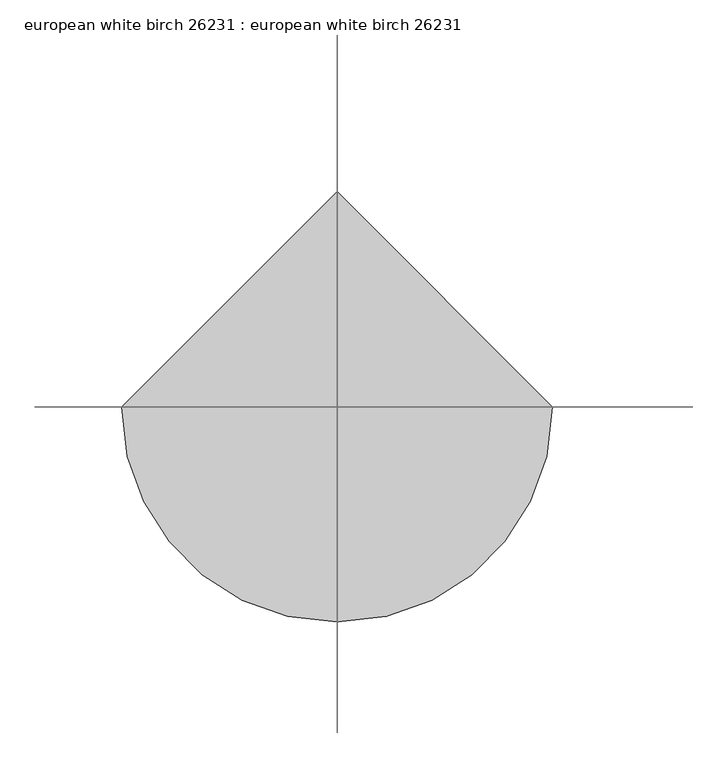
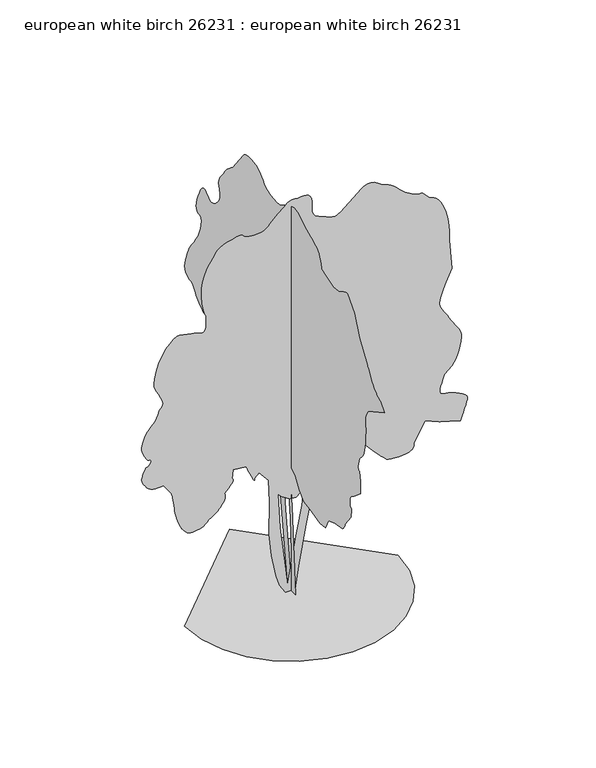
"""IFC4 building model written with IfcOpenShell, lengths in millimetres: proxy geometry, european white birch 26231 : european white birch 26231."""

import ifcopenshell
import ifcopenshell.guid

model = None  # the IFC model being written
_history = None  # IfcOwnerHistory: only IFC2X3 demands one
_inside = {}  # id of a spatial element -> (the spatial element, [elements in it])
_under = {}  # id of a project, library or spatial element -> (it, [spatial elements below it])
_declared = {}  # id of a project -> (the project, [libraries it declares])
_typed = {}  # id of a type object -> (the type object, [elements of that type])
_made_of = {}  # id of a material, layer set ... -> (it, [elements and type objects made of it])


def new_model(schema):
    """Start an empty IFC model of exactly this schema.

    Asked for "IFC4X3", IfcOpenShell would pick the latest addendum, in which some entities
    have other attributes; the version numbers below select the first issue.
    IFC2X3 requires an IfcOwnerHistory on every rooted entity: one is made here for all.
    """
    global model, _history
    if schema == "IFC4X3":
        model = ifcopenshell.file(schema_version=(4, 3, 0, 0))
    else:
        model = ifcopenshell.file(schema=schema)
    _inside.clear()
    _under.clear()
    _declared.clear()
    _typed.clear()
    _made_of.clear()
    _history = None
    if model.schema == "IFC2X3":
        org = make("IfcOrganization", Name="unknown")
        user = make(
            "IfcPersonAndOrganization",
            ThePerson=make("IfcPerson", FamilyName="unknown"),
            TheOrganization=org,
        )
        app = make(
            "IfcApplication",
            ApplicationDeveloper=org,
            Version="unknown",
            ApplicationFullName="unknown",
            ApplicationIdentifier="unknown",
        )
        _history = make(
            "IfcOwnerHistory",
            OwningUser=user,
            OwningApplication=app,
            ChangeAction="ADDED",
            CreationDate=0,
        )
    return model


def make(cls, **values):
    """One entity of the class cls with the attributes given. An attribute that is None is left unset."""
    return model.create_entity(
        cls, **{name: value for name, value in values.items() if value is not None}
    )


def rooted(cls, **values):
    """An entity with a GlobalId (a new one), such as an element, a storey or a relation."""
    return make(cls, GlobalId=ifcopenshell.guid.new(), OwnerHistory=_history, **values)


def si_unit(unit_type, name, prefix=None):
    """IfcSIUnit, for example si_unit("LENGTHUNIT", "METRE", prefix="MILLI")."""
    return make("IfcSIUnit", UnitType=unit_type, Prefix=prefix, Name=name)


def assignment(units):
    """IfcUnitAssignment: the units of a project."""
    return None if units is None else make("IfcUnitAssignment", Units=units)


def point(xyz):
    """IfcCartesianPoint."""
    return None if xyz is None else make("IfcCartesianPoint", Coordinates=xyz)


def direction(xyz):
    """IfcDirection."""
    return None if xyz is None else make("IfcDirection", DirectionRatios=xyz)


def frame(location, z_axis=None, x_axis=None):
    """IfcAxis2Placement3D, a coordinate frame: its origin and axes. An axis left out is left unset."""
    return make(
        "IfcAxis2Placement3D",
        Location=point(location),
        Axis=direction(z_axis),
        RefDirection=direction(x_axis),
    )


def origin():
    """The frame at (0, 0, 0) with its axes left unset."""
    return frame((0.0, 0.0, 0.0))


def place(relative_to, where):
    """IfcLocalPlacement: puts the frame where relative to a parent placement (None: the world)."""
    return make(
        "IfcLocalPlacement", PlacementRelTo=relative_to, RelativePlacement=where
    )


def context(
    kind, dimensions, precision=None, world=None, true_north=None, identifier=None
):
    """IfcGeometricRepresentationContext, for example the 3D "Model" context."""
    return make(
        "IfcGeometricRepresentationContext",
        ContextIdentifier=identifier,
        ContextType=kind,
        CoordinateSpaceDimension=dimensions,
        Precision=precision,
        WorldCoordinateSystem=world,
        TrueNorth=true_north,
    )


def project(units=None, contexts=None):
    """IfcProject with its units and contexts."""
    return rooted(
        "IfcProject",
        Name="project",
        RepresentationContexts=contexts,
        UnitsInContext=assignment(units),
    )


def spatial(cls, under=None, at=None, **own):
    """A site, building, storey or space (cls), placed at a placement, below another one or the project."""
    s = rooted(cls, ObjectPlacement=at, **own)
    if under is not None:
        _under.setdefault(under.id(), (under, []))[1].append(s)
    return s


def point_list(points):
    """IfcCartesianPointList2D or 3D."""
    cls = (
        "IfcCartesianPointList2D" if len(points[0]) == 2 else "IfcCartesianPointList3D"
    )
    return make(cls, CoordList=points)


def triangles(points, corners, closed=None, point_numbers=None):
    """IfcTriangulatedFaceSet: each triangle names its three corners, points numbered from 1."""
    return make(
        "IfcTriangulatedFaceSet",
        Coordinates=point_list(points),
        Closed=closed,
        CoordIndex=corners,
        PnIndex=point_numbers,
    )


def shape(context_of_items, identifier, shape_type, items):
    """IfcShapeRepresentation: the items that make up one representation, for example the "Body"."""
    return make(
        "IfcShapeRepresentation",
        ContextOfItems=context_of_items,
        RepresentationIdentifier=identifier,
        RepresentationType=shape_type,
        Items=items,
    )


def source(mapping_origin, context_of_items, identifier, shape_type, items):
    """IfcRepresentationMap: a shape defined once, which mapped items show again and again."""
    return make(
        "IfcRepresentationMap",
        MappingOrigin=mapping_origin,
        MappedRepresentation=shape(context_of_items, identifier, shape_type, items),
    )


def transform(
    local_origin,
    x_axis=None,
    y_axis=None,
    z_axis=None,
    scale=None,
    scale2=None,
    scale3=None,
    uniform=True,
):
    """IfcCartesianTransformationOperator3D, or its non-uniform kind. x_axis, y_axis, z_axis: its Axis1, 2, 3."""
    if uniform:
        return make(
            "IfcCartesianTransformationOperator3D",
            Axis1=direction(x_axis),
            Axis2=direction(y_axis),
            LocalOrigin=point(local_origin),
            Scale=scale,
            Axis3=direction(z_axis),
        )
    return make(
        "IfcCartesianTransformationOperator3DnonUniform",
        Axis1=direction(x_axis),
        Axis2=direction(y_axis),
        LocalOrigin=point(local_origin),
        Scale=scale,
        Axis3=direction(z_axis),
        Scale2=scale2,
        Scale3=scale3,
    )


def mapped(mapping_source, mapping_target):
    """IfcMappedItem: shows the shape of a source again, moved by a transform."""
    return make(
        "IfcMappedItem", MappingSource=mapping_source, MappingTarget=mapping_target
    )


def made_of(thing, what):
    """Note that an element or type object is made of a material, layer set ...; save() writes the relation."""
    if what is not None:
        _made_of.setdefault(what.id(), (what, []))[1].append(thing)
    return thing


def element(
    cls,
    number,
    at=None,
    inside=None,
    cuts=None,
    type_object=None,
    material=None,
    context=None,
    identifier="Body",
    shape_type=None,
    held_by="IfcProductDefinitionShape",
    body=None,
    shapes=None,
    **own,
):
    """One element of the class cls, such as IfcWall. Its Tag is "e" and its number.

    at: its placement. inside: the storey or other place that contains it. cuts: it is an
    opening in that element (IfcRelVoidsElement). A single representation is given by context,
    identifier, shape_type and body (its items); several are given by shapes. held_by: the class
    of the entity that holds the representations. save() writes the other relations.
    """
    e = rooted(cls, Tag="e%d" % number, ObjectPlacement=at, **own)
    if body is not None:
        shapes = [shape(context, identifier, shape_type, body)]
    if shapes is not None:
        e.Representation = make(held_by, Representations=shapes)
    if inside is not None:
        _inside.setdefault(inside.id(), (inside, []))[1].append(e)
    if cuts is not None:
        rooted(
            "IfcRelVoidsElement", RelatingBuildingElement=cuts, RelatedOpeningElement=e
        )
    if type_object is not None:
        _typed.setdefault(type_object.id(), (type_object, []))[1].append(e)
    return made_of(e, material)


def aggregate(whole, parts):
    """IfcRelAggregates: a whole, such as a stair, and the parts it consists of."""
    return rooted("IfcRelAggregates", RelatingObject=whole, RelatedObjects=parts)


def save(model, path):
    """Write the relations noted so far, then the file.

    IfcRelAggregates (storeys below a building ...), IfcRelContainedInSpatialStructure (elements
    in a storey), IfcRelDefinesByType, IfcRelAssociatesMaterial and IfcRelDeclares: one each for
    every whole, place, type object, material and project.
    """
    for whole, parts in _under.values():
        aggregate(whole, parts)
    for where, things in _inside.values():
        rooted(
            "IfcRelContainedInSpatialStructure",
            RelatedElements=things,
            RelatingStructure=where,
        )
    for kind, things in _typed.values():
        rooted("IfcRelDefinesByType", RelatedObjects=things, RelatingType=kind)
    for what, things in _made_of.values():
        rooted("IfcRelAssociatesMaterial", RelatedObjects=things, RelatingMaterial=what)
    for by, libraries in _declared.values():
        rooted("IfcRelDeclares", RelatingContext=by, RelatedDefinitions=libraries)
    model.write(path)


def european_white_birch_26231_european_white_birch_26231_e71fde4f(model_context):
    return source(origin(), model_context, "Body", "Tessellation", [
        triangles([(27.394651, 0.0040504, 0.0028461), (-40.6021365, 0.0040504, 0.0028461), (-85.9329906, 0.0040461, 71.7768143), (-112.3759078, 0.0040411, 154.8832968), (-146.3742959, 0.004031, 324.873484), (-165.2619874, 0.0040206, 498.6424559), (-161.4844927, 0.004006, 744.1841543), (-169.039464, 0.0039956, 917.9531261), (-237.036004, 0.0039907, 1001.059318), (-271.0331294, 0.0039925, 970.840959), (-270.3066839, 0.0039929, 963.7695883), (-270.075557, 0.0039933, 957.9860023), (-270.8350129, 0.0039934, 954.7830729), (-273.0829134, 0.0039934, 955.4434977), (-277.3120158, 0.0039931, 961.2575323), (-284.0176021, 0.0039923, 973.5155777), (-293.700078, 0.0039911, 993.5053459), (-303.821971, 0.0039898, 1015.3671656), (-311.7620024, 0.0039888, 1032.8676962), (-317.8859382, 0.003988, 1046.7335649), (-322.5544759, 0.0039873, 1057.6911083), (-326.1333272, 0.0039868, 1066.4693516), (-328.985733, 0.0039864, 1073.7921604), (-331.4749343, 0.0039859, 1080.3885601), (-429.6916137, 0.0039853, 1091.7220253), (-437.2481292, 0.0039893, 1023.7262484), (-433.293356, 0.0039894, 1022.0295496), (-429.9024656, 0.0039896, 1019.8705244), (-427.631674, 0.0039898, 1016.7869917), (-427.0500235, 0.00399, 1012.316625), (-428.7111866, 0.0039904, 1005.9945545), (-433.1841331, 0.0039909, 997.3610699), (-441.0251152, 0.0039916, 985.9513739), (-450.1868743, 0.0039923, 973.9905487), (-458.3606123, 0.0039929, 963.8127542), (-465.7062758, 0.0039934, 955.1234591), (-472.3915509, 0.0039939, 947.6228268), (-478.5815437, 0.0039942, 941.0162533), (-484.4387807, 0.0039946, 935.0015768), (-490.1334549, 0.003995, 929.2865913), (-488.5815147, 0.0039955, 919.5735941), (-487.4232642, 0.0039961, 909.8581261), (-487.0600596, 0.0039967, 900.1451288), (-487.8880978, 0.0039973, 890.4322042), (-490.2985611, 0.0039979, 880.7167362), (-494.6927333, 0.0039984, 871.003739), (-501.4669201, 0.003999, 861.2908144), (-508.8125836, 0.0039996, 851.763271), (-515.365781, 0.0040001, 842.4363693), (-522.1831338, 0.0040007, 833.0409399), (-530.3212998, 0.0040013, 823.3152981), (-540.8394442, 0.0040019, 812.9977592), (-554.7941883, 0.0040026, 801.8192265), (-573.2396831, 0.0040033, 789.5154716), (-592.1829672, 0.0040041, 776.4217941), (-607.7557085, 0.0040048, 763.3916302), (-621.2152067, 0.0040056, 750.9583048), (-633.8135656, 0.0040063, 739.6477306), (-646.8107374, 0.0040068, 729.9880732), (-661.4563551, 0.0040073, 722.5103319), (-679.0128416, 0.0040076, 717.742745), (-697.3389759, 0.0040078, 714.6033291), (-713.6812923, 0.0040079, 712.0582083), (-728.3751629, 0.004008, 710.7044392), (-741.7431696, 0.004008, 711.1337008), (-754.1231552, 0.0040078, 713.9429043), (-765.842716, 0.0040075, 719.7239468), (-777.229521, 0.0040069, 729.0736668), (-788.1109062, 0.0040062, 740.6941784), (-798.1336956, 0.0040055, 753.1071562), (-807.361548, 0.0040047, 766.6428125), (-815.8629187, 0.0040037, 781.6313599), (-823.7064079, 0.0040028, 798.4029379), (-830.9530586, 0.0040016, 817.2929186), (-837.6713259, 0.0040004, 838.6238113), (-843.4955343, 0.0039992, 858.8117506), (-848.1996077, 0.0039982, 875.2328413), (-852.042687, 0.0039973, 889.6727303), (-855.291326, 0.0039965, 903.9119774), (-858.2097525, 0.0039955, 919.7387003), (-861.0621946, 0.0039944, 938.9334589), (-864.1127352, 0.0039929, 963.2844435), (-867.2419773, 0.0039915, 988.1637388), (-870.1706503, 0.0039902, 1008.2856211), (-872.9341444, 0.0039893, 1024.4425564), (-875.5681406, 0.0039885, 1037.4270109), (-878.1005442, 0.0039879, 1048.0315235), (-880.566818, 0.0039873, 1057.0510311), (-883.0001724, 0.0039869, 1065.2781452), (-939.6650276, 0.0039821, 1144.6073874), (-960.6453604, 0.0039822, 1143.9037966), (-981.2295691, 0.0039822, 1143.8250223), (-1001.0212389, 0.0039821, 1145.0035841), (-1019.6216297, 0.0039819, 1148.0668419), (-1036.6370882, 0.0039816, 1153.6396122), (-1051.6713449, 0.0039811, 1162.3517984), (-1064.3255871, 0.0039803, 1174.8282898), (-1074.7447186, 0.0039795, 1188.5290524), (-1083.3781305, 0.0039788, 1200.7108669), (-1090.2945688, 0.0039781, 1211.7014025), (-1095.5600178, 0.0039775, 1221.8335602), (-1099.2379183, 0.003977, 1231.4371891), (-1101.3968708, 0.0039764, 1240.842865), (-1102.1004616, 0.0039758, 1250.3805096), (-1100.4266539, 0.0039751, 1261.9120731), (-1096.1086035, 0.0039743, 1276.0193516), (-1090.2056934, 0.0039734, 1291.1195927), (-1083.7743999, 0.0039725, 1305.6229225), (-1077.8714172, 0.0039718, 1317.9470249), (-1073.5534395, 0.0039713, 1326.5043514), (-1071.8795591, 0.0039711, 1329.7098244), (-1068.9941248, 0.003971, 1330.8324303), (-1061.7475468, 0.0039708, 1334.0708954), (-1052.2555389, 0.0039705, 1339.2246506), (-1042.6289463, 0.0039701, 1346.0979229), (-1034.9860989, 0.0039696, 1354.4899979), (-1031.4402397, 0.003969, 1364.2029224), (-1034.1046846, 0.0039684, 1375.0412144), (-1039.5885796, 0.003968, 1382.3080673), (-1043.7516249, 0.0039679, 1383.6975174), (-1047.5844578, 0.0039679, 1382.5722954), (-1052.0777155, 0.003968, 1382.3080673), (-1058.224506, 0.0039677, 1386.2730869), (-1067.012923, 0.003967, 1397.8376427), (-1079.4360746, 0.0039657, 1420.3699883), (-1091.9252106, 0.0039642, 1445.7800652), (-1100.2513739, 0.003963, 1465.4371502), (-1104.4144192, 0.003962, 1481.9243706), (-1104.4144192, 0.0039611, 1497.8171505), (-1100.2513739, 0.00396, 1515.6910595), (-1091.9252106, 0.0039587, 1538.1268993), (-1079.4360746, 0.0039569, 1567.6974781), (-1064.2798777, 0.0039552, 1597.0701038), (-1048.399815, 0.0039538, 1619.0410011), (-1032.4536953, 0.0039528, 1636.3867447), (-1017.0993999, 0.0039519, 1651.8833279), (-1003.0024406, 0.0039509, 1668.3044186), (-990.8230968, 0.0039497, 1688.4261555), (-981.2193953, 0.0039481, 1715.0224972), (-972.0448826, 0.0039467, 1739.5715801), (-961.9458624, 0.0039458, 1754.6033661), (-952.7714224, 0.0039452, 1764.484013), (-946.3731211, 0.0039446, 1773.5695049), (-944.597648, 0.0039439, 1786.2238197), (-949.3017941, 0.0039427, 1806.8080284), (-962.3294146, 0.0039407, 1839.683202), (-979.0807177, 0.0039386, 1873.8004509), (-993.1903942, 0.0039372, 1898.4714741), (-1003.8609638, 0.003936, 1918.5805664), (-1010.3049019, 0.0039348, 1939.0224873), (-1011.7248007, 0.0039332, 1964.6841476), (-1007.3305922, 0.0039311, 2000.4549294), (-996.3298101, 0.0039281, 2051.2269756), (-977.7827591, 0.0039247, 2108.3871494), (-952.959347, 0.0039217, 2159.268346), (-924.3666155, 0.0039191, 2202.6819752), (-894.5216349, 0.003917, 2237.4394466), (-865.9313742, 0.0039155, 2262.3517342), (-841.1054186, 0.0039147, 2276.2302475), (-822.560911, 0.0039146, 2277.8813095), (-705.4567944, 0.0039161, 2251.4372841), (-691.5452162, 0.0039165, 2245.6562416), (-676.5135029, 0.0039168, 2239.8751991), (-661.5453032, 0.003917, 2236.8678246), (-647.8343668, 0.0039169, 2239.4104019), (-636.5669586, 0.0039162, 2250.281686), (-628.9342123, 0.0039149, 2272.2525833), (-626.1275522, 0.0039128, 2308.1021393), (-626.6101536, 0.0039108, 2340.8655464), (-628.1519199, 0.0039099, 2356.9793884), (-630.8849653, 0.0039094, 2364.3021973), (-634.9362442, 0.003909, 2370.7004986), (-640.4429575, 0.0039082, 2384.0379112), (-647.5371466, 0.0039066, 2412.1786354), (-656.3459112, 0.0039035, 2462.9810577), (-661.9085077, 0.0038998, 2524.9316368), (-660.1355782, 0.0038965, 2581.121521), (-652.4800135, 0.0038935, 2631.3882202), (-640.3997915, 0.0038909, 2675.5079109), (-625.3451872, 0.0038886, 2713.2524094), (-608.7691641, 0.0038868, 2744.4943977), (-592.1271203, 0.0038853, 2768.9545326), (-577.5017776, 0.0038841, 2789.7061729), (-564.8602163, 0.0038829, 2809.5183357), (-552.480267, 0.0038818, 2827.9332001), (-538.6474268, 0.0038808, 2844.519397), (-521.6421421, 0.00388, 2858.7688179), (-499.7473303, 0.0038793, 2870.2750923), (-471.2460176, 0.0038788, 2878.5045319), (-442.3357547, 0.0038784, 2885.0579109), (-419.4402045, 0.003878, 2891.1537598), (-401.1674463, 0.0038777, 2895.8528915), (-386.135733, 0.0038776, 2898.2405365), (-372.9506003, 0.0038776, 2897.4022156), (-360.2302649, 0.0038779, 2892.3984512), (-346.5853855, 0.0038786, 2882.2891846), (-328.0611892, 0.0038792, 2871.5959419), (-303.3901842, 0.0038796, 2865.1951698), (-275.2190476, 0.0038797, 2862.7566559), (-246.1878799, 0.0038796, 2863.9757675), (-218.9407967, 0.0038794, 2868.471714), (-196.1211867, 0.0038789, 2875.9392815), (-180.3721843, 0.0038783, 2886.0738373), (-168.3897398, 0.0038776, 2898.2405365), (-155.2838538, 0.0038768, 2911.7277946), (-141.3189358, 0.0038759, 2926.0280846), (-126.7594139, 0.0038751, 2940.5568489), (-111.8694252, 0.0038742, 2954.8571388), (-96.9134068, 0.0038734, 2968.344397), (-82.1555049, 0.0038727, 2980.5110962), (-68.1573178, 0.003872, 2992.5760574), (-54.8202912, 0.0038712, 3005.3776016), (-41.4169714, 0.0038705, 3017.7727753), (-27.2206609, 0.0038698, 3028.6694939), (-11.5045701, 0.0038693, 3036.8989334), (6.4582013, 0.0038691, 3041.3693001), (27.394651, 0.0038691, 3040.9629295), (49.9498399, 0.0038692, 3039.6420799), (71.8443792, 0.0038691, 3040.7344551), (92.4173513, 0.003869, 3041.9535667), (111.007859, 0.0038691, 3041.0390877), (126.954987, 0.0038694, 3035.7812691), (139.5983468, 0.0038701, 3023.8942039), (148.2767597, 0.0038713, 3003.1678528), (152.1975051, 0.0038729, 2976.7517326), (152.8144732, 0.0038745, 2949.9039528), (152.8363106, 0.0038761, 2923.6913086), (154.9729534, 0.0038776, 2899.0276978), (161.9335751, 0.0038789, 2876.9552078), (176.4270581, 0.00388, 2858.4641853), (201.1628484, 0.0038808, 2844.519397), (230.392387, 0.0038815, 2832.759359), (256.9132791, 0.0038822, 2821.2022156), (281.2515464, 0.0038828, 2811.4231613), (303.9388244, 0.0038832, 2804.9971001), (325.5034238, 0.0038833, 2803.5492233), (346.4736554, 0.0038829, 2808.6291458), (367.3752866, 0.0038822, 2821.8626404), (518.4798351, 0.0038745, 2950.2850342), (522.0028032, 0.0038744, 2952.6726791), (531.8706965, 0.003874, 2958.2098412), (547.0243501, 0.0038737, 2964.5597443), (566.409613, 0.0038734, 2969.309745), (588.9648133, 0.0038733, 2970.1224861), (613.6332567, 0.0038737, 2964.5597443), (639.3609015, 0.0038745, 2950.2850342), (662.9625858, 0.0038755, 2934.3845512), (682.9295357, 0.0038761, 2923.8183357), (700.7171127, 0.0038765, 2916.096714), (717.7757372, 0.003877, 2908.7053047), (735.5633869, 0.0038775, 2899.1294357), (755.5303368, 0.0038784, 2884.8800148), (779.1320211, 0.0038797, 2863.4170807), (802.6904669, 0.003881, 2840.7347443), (822.3475519, 0.0038821, 2823.6151497), (839.2969534, 0.0038828, 2810.6612892), (854.7274069, 0.0038834, 2800.5011536), (869.8277206, 0.0038839, 2791.7130272), (885.7865576, 0.0038845, 2782.9246101), (903.7925806, 0.0038851, 2772.7391853), (921.1153605, 0.0038856, 2764.6873512), (935.0701773, 0.0038857, 2761.4360962), (946.9090622, 0.0038858, 2760.445459), (957.8894966, 0.0038859, 2759.1246094), (969.2661278, 0.0038861, 2754.908297), (982.2963644, 0.0038867, 2745.1801117), (998.2323103, 0.0038878, 2727.4000923), (1015.8421366, 0.0038888, 2709.5947838), (1033.1877348, 0.0038895, 2698.6471962), (1050.4673487, 0.00389, 2690.3415985), (1067.8790766, 0.0038906, 2680.4608063), (1085.6209442, 0.0038915, 2664.7382195), (1103.8937387, 0.0038931, 2639.0081039), (1122.890399, 0.0038954, 2598.9776985), (1139.5654713, 0.0038982, 2552.2671776), (1151.2850321, 0.0039008, 2508.9526703), (1158.8719963, 0.0039032, 2468.4345039), (1163.1569818, 0.0039055, 2430.1618401), (1164.9629036, 0.0039077, 2393.5757011), (1165.1152925, 0.0039098, 2358.1121681), (1164.4447666, 0.0039119, 2323.2125542), (1183.3322039, 0.0039254, 2096.5583656), (1160.8760891, 0.0039282, 2049.0019661), (1139.6746943, 0.003931, 2002.6697651), (1120.9853554, 0.0039336, 1958.7811649), (1106.0628651, 0.003936, 1918.5603642), (1096.1619432, 0.0039381, 1883.2289452), (1092.5373825, 0.0039398, 1854.0112518), (1096.4489897, 0.0039411, 1832.1266865), (1105.2043419, 0.0039422, 1814.483868), (1115.1484297, 0.0039432, 1796.9070339), (1126.0856981, 0.0039443, 1778.9975166), (1137.8154327, 0.0039454, 1760.364061), (1150.1394625, 0.0039466, 1740.6053833), (1162.8597616, 0.0039479, 1719.327903), (1175.7782318, 0.0039492, 1696.1351326), (1190.083536, 0.0039507, 1672.4673912), (1206.0423002, 0.003952, 1649.7243027), (1222.0671215, 0.0039534, 1627.4433952), (1236.5705967, 0.0039547, 1605.1651039), (1247.9700462, 0.003956, 1582.42187), (1254.6782124, 0.0039574, 1558.7541286), (1255.1075466, 0.0039589, 1533.6996986), (1250.5482319, 0.0039606, 1505.3836945), (1243.6089752, 0.0039625, 1473.6972565), (1234.6884441, 0.0039645, 1440.8220829), (1224.1805099, 0.0039664, 1408.9400173), (1212.4837675, 0.0039681, 1380.2278164), (1199.9971024, 0.0039695, 1356.867469), (1187.1091536, 0.0039704, 1341.0432896), (1175.1508718, 0.003971, 1330.4793995), (1164.9730774, 0.0039716, 1321.3074303), (1156.2837095, 0.0039721, 1313.2887337), (1148.7831499, 0.0039725, 1306.1970154), (1142.1765764, 0.0039729, 1299.7962433), (1136.1618999, 0.0039732, 1293.8602684), (1130.4468418, 0.0039736, 1288.1553841), (1119.2784828, 0.0039753, 1259.9842838), (1109.1032318, 0.0039769, 1232.7706833), (1100.9092552, 0.0039784, 1207.4723728), (1095.6869722, 0.0039797, 1185.0492502), (1094.4322523, 0.0039808, 1166.4589605), (1098.1329712, 0.0039817, 1152.6591488), (1107.7799114, 0.0039821, 1144.6073874), (1119.8855679, 0.0039824, 1140.5992744), (1130.6017742, 0.0039825, 1137.9779955), (1140.3909296, 0.0039826, 1136.2812241), (1149.7203747, 0.0039827, 1135.0493225), (1159.0472763, 0.0039828, 1133.8148775), (1168.8389751, 0.0039829, 1132.1181787), (1179.5551815, 0.003983, 1129.4968998), (1194.774892, 0.0039834, 1124.1121267), (1215.7451237, 0.0039839, 1115.0925465), (1239.4230389, 0.0039846, 1103.4288689), (1262.7705963, 0.0039854, 1090.1142019), (1282.7503361, 0.0039862, 1076.1391829), (1296.3189846, 0.003987, 1062.4917601), (1300.4363205, 0.0039877, 1050.1676577), (1297.6066967, 0.0039886, 1036.4135553), (1292.5953747, 0.0039897, 1018.2957659), (1285.7677391, 0.0039909, 996.5457127), (1277.4848145, 0.0039924, 971.8848633), (1268.1122761, 0.003994, 945.0472572), (1258.0131832, 0.0039957, 916.7542168), (1247.5510311, 0.0039974, 887.732151), (1088.8924742, 0.0039947, 933.063541), (986.8988451, 0.003992, 978.394931), (903.7925806, 0.0040008, 831.069912), (903.6808142, 0.0040014, 821.3899796), (902.9112391, 0.0040019, 811.9056021), (900.8182709, 0.0040025, 802.8200375), (896.744101, 0.004003, 794.328768), (890.0258337, 0.0040035, 786.6300373), (880.0029716, 0.0040039, 779.9244873), (866.0151627, 0.0040042, 774.4050568), (846.3124409, 0.0040044, 770.254656), (821.2578655, 0.0040046, 767.5546755), (793.3610945, 0.0040047, 766.3761137), (765.1340384, 0.0040046, 766.7850277), (739.086355, 0.0040045, 768.8450037), (717.7325712, 0.0040043, 772.6219534), (703.5797287, 0.004004, 778.1845499), (692.3249651, 0.0040034, 786.972967), (678.2940628, 0.0040027, 799.9244293), (661.9491302, 0.0040017, 816.34552), (643.75511, 0.0040005, 835.5402786), (624.1742558, 0.0039993, 856.8178316), (603.6663142, 0.0039979, 879.4848347), (582.698626, 0.0039965, 902.8426386), (568.1063481, 0.0039956, 918.9335169), (553.3794127, 0.0039947, 934.4301001), (538.3909018, 0.0039938, 948.7353315), (523.0061213, 0.0039931, 961.2575323), (507.0904867, 0.0039924, 971.4022619), (490.5169707, 0.003992, 978.5701384), (473.1484815, 0.0039918, 982.1718807), (299.3795278, 0.0039905, 1004.8388111), (220.0505219, 0.0039938, 948.1740286), (186.0526334, 0.0039972, 891.5117168), (159.6097343, 0.0040064, 736.6301823), (110.5011312, 0.0040218, 479.7550186), (53.8375659, 0.00404, 173.7712428), (-25.4914287, 0.0039615, 56.6666174), (38.7268558, 0.003939, 434.4236286), (80.280474, 0.0039269, 638.4135029), (91.61294, 0.0039203, 747.9636475), (91.61294, 0.0039172, 800.8490095), (68.9477628, 0.0039206, 744.1841543), (34.9493702, 0.0039224, 713.9657953), (-14.1591478, 0.0039219, 721.5197674), (-67.0453035, 0.0039199, 755.5176195), (-97.2657018, 0.0039181, 785.738522), (-82.1555049, 0.0039341, 517.5298568), (0.0001483, 43.8182829, 0.0020761), (0.0001483, -54.3986509, 0.0020703), (0.0001483, -9.0678473, 664.8549122), (0.0001483, 13.5975031, 895.2886665), (0.0001483, 28.7078316, 978.394931), (0.0001483, -54.3986509, 925.5070255), (0.0001483, -107.2847305, 846.1777834), (0.0001483, -163.9485502, 793.292494), (0.0001483, -239.5000614, 778.1820065), (0.0001483, -303.7178349, 763.0715916), (0.0001483, -367.9366259, 747.961104), (0.0001483, -439.7119323, 755.5176195), (0.0001483, -473.7098207, 831.069912), (0.0001483, -556.8160489, 861.288271), (0.0001483, -655.032692, 880.1782516), (0.0001483, -659.8892269, 885.0778799), (0.0001483, -664.7482327, 890.2442797), (0.0001483, -669.6046949, 895.9363741), (0.0001483, -674.4611572, 902.4235508), (0.0001483, -679.3176195, 909.9673491), (0.0001483, -684.1741545, 918.8344677), (0.0001483, -689.0306168, 929.2865913), (0.0001483, -695.1011765, 941.3896317), (0.0001483, -703.3485655, 954.8795786), (0.0001483, -713.4145935, 969.5277397), (0.0001483, -724.9360559, 985.100481), (0.0001483, -737.5445887, 1001.3691828), (0.0001483, -750.8821466, 1018.0976675), (0.0001483, -764.5829092, 1035.0571701), (0.0001483, -772.139352, 1099.2759974), (0.0001483, -766.5208723, 1102.6135843), (0.0001483, -761.2021563, 1106.5454664), (0.0001483, -756.4777353, 1111.6660841), (0.0001483, -752.6449024, 1118.5723486), (0.0001483, -750.0007324, 1127.8560843), (0.0001483, -748.8450617, 1140.1141296), (0.0001483, -749.4724216, 1155.9408525), (0.0001483, -752.3045162, 1171.9860214), (0.0001483, -757.3133675, 1184.861253), (0.0001483, -764.1434738, 1195.0923872), (0.0001483, -772.423855, 1203.2102057), (0.0001483, -781.7964661, 1209.7405483), (0.0001483, -791.8954863, 1215.2142694), (0.0001483, -802.357711, 1220.1596798), (0.0001483, -881.6869532, 1288.1553841), (0.0001483, -885.466519, 1390.1490131), (0.0001483, -870.3560314, 1458.1473335), (0.0001483, -864.7832611, 1459.9406834), (0.0001483, -859.7718664, 1462.7929802), (0.0001483, -855.8831503, 1467.7612816), (0.0001483, -853.6809591, 1475.8994476), (0.0001483, -853.7241251, 1488.266716), (0.0001483, -856.5765673, 1505.922179), (0.0001483, -862.7995886, 1529.9201328), (0.0001483, -870.719236, 1551.8250458), (0.0001483, -878.5043713, 1565.0076714), (0.0001483, -886.4901484, 1573.2347855), (0.0001483, -895.0042362, 1580.2730186), (0.0001483, -904.3742311, 1589.8869667), (0.0001483, -914.9381212, 1605.845731), (0.0001483, -927.0183432, 1631.9137619), (0.0001483, -937.5923344, 1663.1050266), (0.0001483, -944.0667938, 1691.78409), (0.0001483, -947.437373, 1717.7529991), (0.0001483, -948.6921656, 1740.8136555), (0.0001483, -948.8242069, 1760.7704315), (0.0001483, -948.8242069, 1777.4227581), (0.0001483, -949.6852736, 1790.5722462), (0.0001483, -951.4683769, 1799.6908756), (0.0001483, -953.3200081, 1805.7056248), (0.0001483, -954.8389561, 1810.5951519), (0.0001483, -955.6314222, 1816.3430569), (0.0001483, -955.3012098, 1824.9333755), (0.0001483, -953.4521221, 1838.3497078), (0.0001483, -949.6852736, 1858.5705666), (0.0001483, -946.70079, 1881.7531631), (0.0001483, -947.0843422, 1902.9520145), (0.0001483, -950.2796413, 1922.50242), (0.0001483, -955.7203703, 1940.7293598), (0.0001483, -962.8450081, 1957.9658077), (0.0001483, -971.0949406, 1974.53936), (0.0001483, -979.9036325, 1990.7851707), (0.0001483, -1191.4500223, 2107.8892147), (0.0001483, -1138.5621895, 2164.5515991), (0.0001483, -1128.8162001, 2168.6714058), (0.0001483, -1118.8721123, 2173.2205467), (0.0001483, -1108.5292116, 2178.6282108), (0.0001483, -1097.5944866, 2185.3237324), (0.0001483, -1085.8648247, 2193.7387711), (0.0001483, -1073.1445255, 2204.300045), (0.0001483, -1059.2329473, 2217.4395046), (0.0001483, -1043.7160892, 2235.2574577), (0.0001483, -1027.1399935, 2257.7696011), (0.0001483, -1010.7646849, 2282.2627281), (0.0001483, -995.8421946, 2306.029446), (0.0001483, -983.6273151, 2326.3596004), (0.0001483, -975.3773827, 2340.5455078), (0.0001483, -972.3497332, 2345.8770138), (0.0001483, -870.3560314, 2496.9789825), (0.0001483, -809.9142265, 2651.8605171), (0.0001483, -715.4745695, 2746.297776), (0.0001483, -714.1080105, 2746.4248032), (0.0001483, -710.0998976, 2746.4248032), (0.0001483, -703.5797287, 2745.7135094), (0.0001483, -694.6820887, 2743.6560768), (0.0001483, -683.5366207, 2739.6938187), (0.0001483, -670.2752209, 2733.2165977), (0.0001483, -655.032692, 2723.6410194), (0.0001483, -638.8427645, 2713.734938), (0.0001483, -622.6553804, 2706.4196869), (0.0001483, -606.4653803, 2701.2380264), (0.0001483, -590.2754528, 2697.7835861), (0.0001483, -574.085489, 2695.5994171), (0.0001483, -557.8955252, 2694.3038567), (0.0001483, -541.7055977, 2693.4149574), (0.0001483, -447.265868, 2716.071714), (0.0001483, -390.6035926, 2734.9693977), (0.0001483, -389.2700984, 2739.8714241), (0.0001483, -385.4931124, 2752.9017334), (0.0001483, -379.6003035, 2771.5453629), (0.0001483, -371.9244275, 2793.2876404), (0.0001483, -362.7931171, 2815.6397644), (0.0001483, -352.541708, 2836.0611923), (0.0001483, -341.4952529, 2852.0631226), (0.0001483, -328.1907234, 2864.4077179), (0.0001483, -311.3835734, 2875.7360962), (0.0001483, -291.7366622, 2886.4549187), (0.0001483, -269.9079074, 2896.995845), (0.0001483, -246.5594779, 2907.7399567), (0.0001483, -222.3522709, 2919.068335), (0.0001483, -197.946693, 2931.4129303), (0.0001483, -172.8141609, 2945.8655365), (0.0001483, -146.2940319, 2961.968914), (0.0001483, -118.8488412, 2977.6915009), (0.0001483, -90.941106, 2990.9502846), (0.0001483, -63.0331211, 2999.7387016), (0.0001483, -35.5879259, 3001.9740303), (0.0001483, -9.0678473, 2995.6241272), (0.0001483, 15.5359294, 2984.4989342), (0.0001483, 37.8929746, 2973.7039536), (0.0001483, 58.5319923, 2963.1121582), (0.0001483, 77.9815228, 2952.5709412), (0.0001483, 96.7704014, 2941.9791458), (0.0001483, 115.4269479, 2931.1841652), (0.0001483, 134.479991, 2920.0589722), (0.0001483, 158.8525495, 2912.4135086), (0.0001483, 190.6921939, 2911.194397), (0.0001483, 226.364199, 2914.9028915), (0.0001483, 262.2345749, 2922.1416939), (0.0001483, 294.6678241, 2931.4129303), (0.0001483, 320.0322461, 2941.2681427), (0.0001483, 334.690581, 2950.2850342), (0.0001483, 345.0334454, 2961.4610962), (0.0001483, 359.6029049, 2977.2598412), (0.0001483, 378.0077408, 2995.3953621), (0.0001483, 399.8466331, 3013.5055939), (0.0001483, 424.7259284, 3029.3043388), (0.0001483, 452.246814, 3040.4804008), (0.0001483, 482.0181436, 3044.7222931), (0.0001483, 509.7701923, 3045.6111923), (0.0001483, 532.4371227, 3047.2366745), (0.0001483, 551.4007545, 3047.9988373), (0.0001483, 568.0530084, 3046.3224861), (0.0001483, 583.7806821, 3040.607428), (0.0001483, 599.9706096, 3029.2534698), (0.0001483, 618.0096611, 3010.7368675), (0.0001483, 742.6702932, 2848.3040497), (0.0001483, 753.8818909, 2837.2805946), (0.0001483, 767.6029284, 2826.4091652), (0.0001483, 783.1096127, 2814.9031815), (0.0001483, 799.6755346, 2801.8981613), (0.0001483, 816.5690529, 2786.683683), (0.0001483, 833.0663017, 2768.3955551), (0.0001483, 848.4409447, 2746.297776), (0.0001483, 862.736075, 2724.5807877), (0.0001483, 876.3047235, 2707.0801117), (0.0001483, 888.8828075, 2692.4751892), (0.0001483, 900.2035555, 2679.4704597), (0.0001483, 910.0054281, 2666.7194939), (0.0001483, 918.0241974, 2652.9273125), (0.0001483, 923.9932371, 2636.7474861), (0.0001483, 925.4028894, 2616.8085869), (0.0001483, 921.857103, 2593.3896675), (0.0001483, 916.2614416, 2567.5581047), (0.0001483, 911.5269196, 2540.4815598), (0.0001483, 910.5566299, 2513.2907776), (0.0001483, 916.2614416, 2487.0781334), (0.0001483, 931.5471365, 2462.9810577), (0.0001483, 951.2956404, 2442.8058357), (0.0001483, 968.7962437, 2427.385556), (0.0001483, 984.5772572, 2416.3949478), (0.0001483, 999.1695351, 2409.5014732), (0.0001483, 1013.1014608, 2406.3721584), (0.0001483, 1026.9012726, 2406.6820232), (0.0001483, 1041.0973537, 2410.0957684), (0.0001483, 1055.7023489, 2418.4549965), (0.0001483, 1070.502899, 2431.1752956), (0.0001483, 1085.7022619, 2444.2917915), (0.0001483, 1101.4959927, 2453.8397552), (0.0001483, 1118.0821169, 2455.8564926), (0.0001483, 1135.658951, 2446.3745132), (0.0001483, 1154.424448, 2421.4292336), (0.0001483, 1172.6082945, 2386.9666569), (0.0001483, 1187.9498726, 2352.5064056), (0.0001483, 1199.9209442, 2319.4331337), (0.0001483, 1207.9930532, 2289.1360004), (0.0001483, 1211.640505, 2263.0019852), (0.0001483, 1210.3298292, 2242.4177765), (0.0001483, 1203.5327877, 2228.7729698), (0.0001483, 1192.4761951, 2222.4051899), (0.0001483, 1179.8345976, 2220.4010971), (0.0001483, 1167.2565136, 2219.2555275), (0.0001483, 1156.3980194, 2215.468404), (0.0001483, 1148.9075609, 2205.5344173), (0.0001483, 1146.4412144, 2185.9510197), (0.0001483, 1150.6474983, 2153.2206047), (0.0001483, 1159.9972183, 2115.6438286), (0.0001483, 1171.3306835, 2083.4164352), (0.0001483, 1183.8528843, 2055.8852669), (0.0001483, 1196.7713545, 2032.382777), (0.0001483, 1209.2934826, 2012.2481049), (0.0001483, 1220.6269478, 1994.8263485), (0.0001483, 1229.9766678, 1979.4517056), (0.0001483, 1240.3526333, 1963.1729027), (0.0001483, 1254.2286758, 1944.0543022), (0.0001483, 1270.0223339, 1922.9544273), (0.0001483, 1286.1462044, 1900.7294758), (0.0001483, 1301.0128841, 1878.2402962), (0.0001483, 1313.0397663, 1856.345557), (0.0001483, 1320.6394478, 1835.9036362), (0.0001483, 1327.6548626, 1813.7878349), (0.0001483, 1337.4440907, 1787.5776615), (0.0001483, 1347.6981159, 1759.1854992), (0.0001483, 1356.1029808, 1730.5292542), (0.0001483, 1360.3421116, 1703.5239258), (0.0001483, 1358.1069283, 1680.0874203), (0.0001483, 1347.0808571, 1662.134737), (0.0001483, 1331.1449112, 1650.1204994), (0.0001483, 1315.8032604, 1642.3328934), (0.0001483, 1301.1881641, 1637.45354), (0.0001483, 1287.4340618, 1634.1617352), (0.0001483, 1274.6679806, 1631.134013), (0.0001483, 1263.0272667, 1627.0471985), (0.0001483, 1252.6411274, 1620.5829128), (0.0001483, 1244.3708473, 1612.653019), (0.0001483, 1238.27994, 1604.7891094), (0.0001483, 1233.3142548, 1596.5951328), (0.0001483, 1228.4120831, 1587.6746017), (0.0001483, 1222.5218903, 1577.628994), (0.0001483, 1214.5792791, 1566.066909), (0.0001483, 1203.5327877, 1552.5845924), (0.0001483, 1190.6930918, 1539.1175365), (0.0001483, 1178.0490234, 1527.6289936), (0.0001483, 1165.5699886, 1517.7941288), (0.0001483, 1153.2256113, 1509.2801136), (0.0001483, 1140.9777397, 1501.7592064), (0.0001483, 1128.7983959, 1494.8985786), (0.0001483, 1116.6495735, 1488.3656925), (0.0001483, 1094.9198679, 1495.4802292), (0.0001483, 1073.9521797, 1501.5711365), (0.0001483, 1054.5008961, 1505.6149303), (0.0001483, 1037.3305052, 1506.5826038), (0.0001483, 1023.200481, 1503.4559052), (0.0001483, 1012.8702976, 1495.2059727), (0.0001483, 1007.0994289, 1480.8117931), (0.0001483, 1005.2935072, 1464.103656), (0.0001483, 1006.0656258, 1449.3792641), (0.0001483, 1008.9841249, 1436.3059341), (0.0001483, 1013.6195978, 1424.5559246), (0.0001483, 1019.5453989, 1413.7964069), (0.0001483, 1026.3297958, 1403.6974594), (0.0001483, 1033.5433817, 1393.9285789), (0.0001483, 1045.6134298, 1385.8005867), (0.0001483, 1057.2542891, 1377.4744961), (0.0001483, 1068.0365524, 1368.7520634), (0.0001483, 1077.5311037, 1359.4328648), (0.0001483, 1085.3059925, 1349.3235981), (0.0001483, 1090.934646, 1338.2213688), (0.0001483, 1093.9851866, 1325.9302586), (0.0001483, 1099.3597858, 1310.8528358), (0.0001483, 1110.6145494, 1292.2753361), (0.0001483, 1125.3058765, 1271.3152782), (0.0001483, 1140.9878408, 1249.1029713), (0.0001483, 1155.2194576, 1226.7560795), (0.0001483, 1165.549641, 1205.402223), (0.0001483, 1169.5349356, 1186.161755), (0.0001483, 1170.7134974, 1164.7850801), (0.0001483, 1173.4134779, 1137.7239412), (0.0001483, 1176.3751431, 1107.1627253), (0.0001483, 1178.346171, 1075.2781162), (0.0001483, 1178.0718418, 1044.2545738), (0.0001483, 1174.2923487, 1016.2688547), (0.0001483, 1165.7579132, 993.5053459), (0.0001483, 1155.8900562, 976.9065044), (0.0001483, 1148.3360842, 965.2656452), (0.0001483, 1142.1664026, 957.5237486), (0.0001483, 1136.461591, 952.6240477), (0.0001483, 1130.2944529, 949.5049793), (0.0001483, 1122.7404808, 947.1173344), (0.0001483, 1112.8726238, 944.3970062), (0.0001483, 1102.430674, 943.3505585), (0.0001483, 1093.6422569, 945.275877), (0.0001483, 1086.3067308, 948.0622622), (0.0001483, 1080.2285408, 949.5938547), (0.0001483, 1075.2069723, 947.7548681), (0.0001483, 1071.043927, 940.4320593), (0.0001483, 1067.5412338, 925.5070255), (0.0001483, 1064.4805195, 907.1809639), (0.0001483, 1061.5493757, 890.8385748), (0.0001483, 1058.422677, 876.1472477), (0.0001483, 1054.7650515, 862.7766975), (0.0001483, 1050.2489754, 850.3967119), (0.0001483, 1044.544091, 838.6796946), (0.0001483, 1037.3203314, 827.2903461), (0.0001483, 1027.9045544, 814.7808626), (0.0001483, 1016.1088354, 800.7498877), (0.0001483, 1002.331842, 786.45483), (0.0001483, 986.9673729, 773.1502642), (0.0001483, 970.4142408, 762.0911282), (0.0001483, 953.0685699, 754.5371561), (0.0001483, 935.3267023, 751.7406698), (0.0001483, 913.4547815, 757.3895983), (0.0001483, 885.700153, 771.9590578), (0.0001483, 855.4360846, 791.882769), (0.0001483, 826.0305393, 813.5895836), (0.0001483, 800.8540237, 833.5133675), (0.0001483, 783.2747189, 848.0853704), (0.0001483, 776.668218, 853.7342989), (0.0001483, 772.4619341, 859.0429138), (0.0001483, 761.5145645, 872.1493086), (0.0001483, 746.3380926, 888.8218374), (0.0001483, 729.4419582, 904.8365576), (0.0001483, 713.3409061, 915.9592072), (0.0001483, 700.5444489, 917.9632273), (0.0001483, 693.5619535, 906.6195883), (0.0001483, 693.1657568, 889.1647671), (0.0001483, 696.8639322, 874.2854427), (0.0001483, 702.2843136, 859.9344292), (0.0001483, 707.0417267, 844.0645403), (0.0001483, 708.758773, 824.6259012), (0.0001483, 705.0579815, 799.5713259), (0.0001483, 693.5619535, 766.8510847), (0.0001483, 679.8942558, 733.8209787), (0.0001483, 670.2574894, 708.4565386), (0.0001483, 663.1302355, 689.6351583), (0.0001483, 656.9961622, 676.2315434), (0.0001483, 650.3337055, 667.1230877), (0.0001483, 641.6215193, 661.1871128), (0.0001483, 629.343199, 657.3009401), (0.0001483, 615.6627113, 655.8125135), (0.0001483, 603.6383726, 657.4329815), (0.0001483, 593.0643451, 661.5630346), (0.0001483, 583.7476536, 667.6082325), (0.0001483, 575.4875836, 674.9768234), (0.0001483, 568.0860005, 683.0717508), (0.0001483, 561.3448422, 691.2987923), (0.0001483, 555.7517607, 702.0354189), (0.0001483, 551.7436478, 717.5319294), (0.0001483, 549.0563481, 736.9933868), (0.0001483, 547.4256701, 759.6247816), (0.0001483, 546.5874581, 784.636191), (0.0001483, 546.2801368, 811.23246), (0.0001483, 546.2369345, 838.6238113), (0.0001483, 553.7909065, 970.8384155), (0.0001483, 602.8992462, 1099.2759974), (0.0001483, 504.6825668, 1186.161755), (0.0001483, 357.3575478, 1193.715727), (0.0001483, 285.5822413, 1103.052947), (0.0001483, 194.9212963, 1016.1698055), (0.0001483, 164.7003938, 876.3986858), (0.0001483, 138.2574766, 664.8549122), (0.0002414, 85.3713969, 989.7258528), (0.0002414, 58.9284843, 936.8404907), (0.0002414, 32.4853173, 793.292494), (0.0002414, 6.0423779, 559.0842607), (0.0002414, -1.5127294, 309.7630328), (0.0002414, 2.264719, 75.5535415), (0.0002414, 70.2612001, 593.0821492), (0.0002414, 126.9247654, 1035.0571701), (-787.0034157, 0.0, 8.68e-05), (-766.1982903, -180.3292545, 7.6e-05), (-706.9426775, -345.9326274, 6.61e-05), (-613.9838167, -492.0663674, 5.74e-05), (-492.0663674, -613.9838167, 5.02e-05), (-345.9326274, -706.9426775, 4.46e-05), (-180.3290002, -766.1982903, 4.11e-05), (3.45e-05, -787.0034157, 3.99e-05), (180.3292545, -766.1982903, 4.11e-05), (345.9326274, -706.9426775, 4.46e-05), (492.0663674, -613.9838167, 5.02e-05), (613.9838167, -492.0663674, 5.74e-05), (706.9426775, -345.9326274, 6.61e-05), (766.1982903, -180.3290002, 7.6e-05), (787.0034157, 6.88e-05, 8.68e-05), (-0.0001035, 787.0034157, 0.0001337)], [[383, 1, 2], [383, 2, 3], [382, 1, 383], [382, 383, 384], [381, 382, 384], [381, 384, 385], [380, 381, 385], [380, 385, 386], [393, 383, 3], [393, 3, 4], [393, 4, 5], [393, 5, 6], [393, 6, 7], [392, 393, 7], [392, 7, 8], [12, 13, 14], [12, 14, 15], [11, 12, 15], [379, 380, 386], [379, 386, 387], [344, 345, 346], [11, 15, 16], [10, 11, 16], [343, 344, 346], [342, 343, 346], [341, 342, 346], [340, 341, 346], [9, 10, 16], [9, 16, 17], [9, 17, 18], [9, 18, 19], [339, 340, 346], [338, 339, 346], [337, 338, 346], [336, 337, 346], [335, 336, 346], [334, 335, 346], [333, 334, 346], [332, 333, 346], [331, 332, 346], [330, 331, 346], [329, 330, 346], [328, 329, 346], [327, 328, 346], [327, 346, 347], [326, 327, 347], [325, 326, 347], [324, 325, 347], [323, 324, 347], [388, 389, 390], [387, 388, 390], [387, 390, 391], [387, 391, 392], [387, 392, 8], [379, 387, 8], [378, 379, 8], [378, 8, 9], [322, 323, 347], [9, 19, 20], [377, 378, 9], [110, 111, 112], [9, 20, 21], [121, 122, 123], [120, 121, 123], [120, 123, 124], [9, 21, 22], [377, 9, 22], [377, 22, 23], [377, 23, 24], [281, 282, 283], [120, 124, 125], [28, 29, 30], [27, 28, 30], [27, 30, 31], [26, 27, 31], [26, 31, 32], [26, 32, 33], [26, 33, 34], [119, 120, 125], [321, 322, 347], [221, 222, 223], [221, 223, 224], [220, 221, 224], [220, 224, 225], [219, 220, 225], [219, 225, 226], [218, 219, 226], [218, 226, 227], [217, 218, 227], [217, 227, 228], [216, 217, 228], [215, 216, 228], [214, 215, 228], [213, 214, 228], [212, 213, 228], [211, 212, 228], [210, 211, 228], [209, 210, 228], [208, 209, 228], [208, 228, 229], [207, 208, 229], [206, 207, 229], [205, 206, 229], [204, 205, 229], [203, 204, 229], [203, 229, 230], [202, 203, 230], [202, 230, 231], [26, 34, 35], [158, 159, 160], [158, 160, 161], [157, 158, 161], [156, 157, 161], [155, 156, 161], [154, 155, 161], [154, 161, 162], [154, 162, 163], [153, 154, 163], [152, 153, 163], [152, 163, 164], [151, 152, 164], [150, 151, 164], [149, 150, 164], [148, 149, 164], [147, 148, 164], [146, 147, 164], [145, 146, 164], [144, 145, 164], [144, 164, 165], [143, 144, 165], [281, 283, 284], [201, 202, 231], [26, 35, 36], [119, 125, 126], [109, 110, 112], [109, 112, 113], [108, 109, 113], [108, 113, 114], [107, 108, 114], [26, 36, 37], [201, 231, 232], [201, 232, 233], [281, 284, 285], [25, 26, 37], [25, 37, 38], [25, 38, 39], [25, 39, 40], [193, 194, 195], [193, 195, 196], [192, 193, 196], [191, 192, 196], [191, 196, 197], [190, 191, 197], [189, 190, 197], [188, 189, 197], [187, 188, 197], [186, 187, 197], [185, 186, 197], [184, 185, 197], [183, 184, 197], [182, 183, 197], [182, 197, 198], [181, 182, 198], [180, 181, 198], [179, 180, 198], [178, 179, 198], [177, 178, 198], [176, 177, 198], [175, 176, 198], [175, 198, 199], [174, 175, 199], [173, 174, 199], [172, 173, 199], [171, 172, 199], [170, 171, 199], [170, 199, 200], [170, 200, 201], [170, 201, 233], [169, 170, 233], [168, 169, 233], [167, 168, 233], [167, 233, 234], [167, 234, 235], [166, 167, 235], [166, 235, 236], [106, 107, 114], [106, 114, 115], [105, 106, 115], [104, 105, 115], [103, 104, 115], [102, 103, 115], [101, 102, 115], [100, 101, 115], [99, 100, 115], [98, 99, 115], [97, 98, 115], [96, 97, 115], [95, 96, 115], [94, 95, 115], [93, 94, 115], [92, 93, 115], [91, 92, 115], [90, 91, 115], [90, 115, 116], [90, 116, 117], [119, 126, 127], [119, 127, 128], [119, 128, 129], [119, 129, 130], [119, 130, 131], [119, 131, 132], [119, 132, 133], [119, 133, 134], [119, 134, 135], [119, 135, 136], [118, 119, 136], [118, 136, 137], [118, 137, 138], [117, 118, 138], [90, 117, 138], [89, 90, 138], [89, 138, 139], [89, 139, 140], [89, 140, 141], [89, 141, 142], [89, 142, 143], [89, 143, 165], [89, 165, 166], [89, 166, 236], [88, 89, 236], [87, 88, 236], [86, 87, 236], [85, 86, 236], [84, 85, 236], [84, 236, 237], [83, 84, 237], [82, 83, 237], [81, 82, 237], [80, 81, 237], [79, 80, 237], [78, 79, 237], [77, 78, 237], [76, 77, 237], [75, 76, 237], [74, 75, 237], [73, 74, 237], [72, 73, 237], [71, 72, 237], [70, 71, 237], [69, 70, 237], [68, 69, 237], [67, 68, 237], [66, 67, 237], [65, 66, 237], [64, 65, 237], [63, 64, 237], [62, 63, 237], [61, 62, 237], [60, 61, 237], [59, 60, 237], [58, 59, 237], [57, 58, 237], [56, 57, 237], [55, 56, 237], [54, 55, 237], [54, 237, 238], [361, 362, 363], [360, 361, 363], [360, 363, 364], [359, 360, 364], [359, 364, 365], [358, 359, 365], [358, 365, 366], [357, 358, 366], [356, 357, 366], [355, 356, 366], [354, 355, 366], [353, 354, 366], [352, 353, 366], [351, 352, 366], [350, 351, 366], [349, 350, 366], [348, 349, 366], [347, 348, 366], [347, 366, 367], [347, 367, 368], [347, 368, 369], [347, 369, 370], [347, 370, 371], [321, 347, 371], [321, 371, 372], [321, 372, 373], [320, 321, 373], [320, 373, 374], [319, 320, 374], [319, 374, 375], [318, 319, 375], [317, 318, 375], [317, 375, 376], [317, 376, 377], [316, 317, 377], [316, 377, 24], [315, 316, 24], [314, 315, 24], [313, 314, 24], [312, 313, 24], [311, 312, 24], [310, 311, 24], [309, 310, 24], [308, 309, 24], [307, 308, 24], [306, 307, 24], [305, 306, 24], [304, 305, 24], [303, 304, 24], [302, 303, 24], [301, 302, 24], [300, 301, 24], [299, 300, 24], [298, 299, 24], [297, 298, 24], [296, 297, 24], [295, 296, 24], [294, 295, 24], [293, 294, 24], [292, 293, 24], [291, 292, 24], [290, 291, 24], [289, 290, 24], [288, 289, 24], [287, 288, 24], [286, 287, 24], [285, 286, 24], [281, 285, 24], [280, 281, 24], [279, 280, 24], [278, 279, 24], [277, 278, 24], [276, 277, 24], [275, 276, 24], [274, 275, 24], [273, 274, 24], [272, 273, 24], [271, 272, 24], [270, 271, 24], [269, 270, 24], [268, 269, 24], [267, 268, 24], [266, 267, 24], [265, 266, 24], [264, 265, 24], [263, 264, 24], [262, 263, 24], [261, 262, 24], [260, 261, 24], [259, 260, 24], [258, 259, 24], [257, 258, 24], [256, 257, 24], [255, 256, 24], [254, 255, 24], [253, 254, 24], [252, 253, 24], [251, 252, 24], [250, 251, 24], [249, 250, 24], [248, 249, 24], [247, 248, 24], [246, 247, 24], [245, 246, 24], [244, 245, 24], [243, 244, 24], [242, 243, 24], [241, 242, 24], [240, 241, 24], [239, 240, 24], [238, 239, 24], [238, 24, 25], [54, 238, 25], [54, 25, 40], [53, 54, 40], [52, 53, 40], [51, 52, 40], [50, 51, 40], [49, 50, 40], [48, 49, 40], [48, 40, 41], [47, 48, 41], [47, 41, 42], [47, 42, 43], [46, 47, 43], [45, 46, 43], [44, 45, 43], [764, 394, 770], [764, 770, 771], [764, 771, 772], [763, 764, 772], [762, 763, 772], [770, 394, 395], [770, 395, 396], [769, 770, 396], [768, 769, 396], [767, 768, 396], [767, 396, 397], [766, 767, 397], [766, 397, 398], [765, 766, 398], [475, 476, 477], [475, 477, 478], [475, 478, 479], [475, 479, 480], [475, 480, 481], [475, 481, 482], [475, 482, 483], [475, 483, 484], [422, 423, 424], [475, 484, 485], [404, 405, 406], [439, 440, 441], [761, 762, 772], [422, 424, 425], [403, 404, 406], [475, 485, 486], [437, 438, 439], [650, 651, 652], [439, 441, 442], [437, 439, 442], [436, 437, 442], [436, 442, 443], [435, 436, 443], [475, 486, 487], [421, 422, 425], [421, 425, 426], [493, 494, 495], [493, 495, 496], [493, 496, 497], [493, 497, 498], [493, 498, 499], [493, 499, 500], [493, 500, 501], [493, 501, 502], [492, 493, 502], [492, 502, 503], [492, 503, 504], [492, 504, 505], [492, 505, 506], [434, 435, 443], [492, 506, 507], [475, 487, 488], [772, 765, 398], [492, 507, 508], [592, 593, 594], [591, 592, 594], [591, 594, 595], [590, 591, 595], [590, 595, 596], [589, 590, 596], [589, 596, 597], [588, 589, 597], [588, 597, 598], [588, 598, 599], [587, 588, 599], [587, 599, 600], [587, 600, 601], [587, 601, 602], [587, 602, 603], [587, 603, 604], [587, 604, 605], [587, 605, 606], [587, 606, 607], [586, 587, 607], [585, 586, 607], [585, 607, 608], [420, 421, 426], [420, 426, 427], [402, 403, 406], [407, 408, 409], [475, 488, 489], [407, 409, 410], [407, 410, 411], [407, 411, 412], [407, 412, 413], [407, 413, 414], [407, 414, 415], [407, 415, 416], [434, 443, 444], [400, 401, 402], [400, 402, 406], [399, 400, 406], [399, 406, 407], [399, 407, 416], [399, 416, 417], [399, 417, 418], [399, 418, 419], [399, 419, 420], [399, 420, 427], [399, 427, 428], [399, 428, 429], [399, 429, 430], [399, 430, 431], [398, 399, 431], [398, 431, 432], [772, 398, 432], [772, 432, 433], [772, 433, 434], [772, 434, 444], [772, 444, 445], [772, 445, 446], [772, 446, 447], [761, 772, 447], [760, 761, 447], [760, 447, 448], [760, 448, 449], [584, 585, 608], [475, 489, 490], [649, 650, 652], [474, 475, 490], [474, 490, 491], [474, 491, 492], [474, 492, 508], [473, 474, 508], [472, 473, 508], [472, 508, 509], [471, 472, 509], [470, 471, 509], [470, 509, 510], [469, 470, 510], [760, 449, 450], [584, 608, 609], [628, 629, 630], [628, 630, 631], [627, 628, 631], [627, 631, 632], [627, 632, 633], [626, 627, 633], [626, 633, 634], [626, 634, 635], [625, 626, 635], [625, 635, 636], [624, 625, 636], [624, 636, 637], [623, 624, 637], [622, 623, 637], [621, 622, 637], [620, 621, 637], [619, 620, 637], [619, 637, 638], [618, 619, 638], [617, 618, 638], [617, 638, 639], [616, 617, 639], [616, 639, 640], [615, 616, 640], [614, 615, 640], [614, 640, 641], [614, 641, 642], [614, 642, 643], [614, 643, 644], [614, 644, 645], [614, 645, 646], [614, 646, 647], [614, 647, 648], [614, 648, 649], [614, 649, 652], [614, 652, 653], [614, 653, 654], [614, 654, 655], [614, 655, 656], [613, 614, 656], [612, 613, 656], [611, 612, 656], [611, 656, 657], [610, 611, 657], [609, 610, 657], [584, 609, 657], [583, 584, 657], [582, 583, 657], [581, 582, 657], [580, 581, 657], [580, 657, 658], [468, 469, 510], [713, 714, 715], [712, 713, 715], [712, 715, 716], [711, 712, 716], [710, 711, 716], [710, 716, 717], [709, 710, 717], [708, 709, 717], [707, 708, 717], [707, 717, 718], [706, 707, 718], [705, 706, 718], [704, 705, 718], [703, 704, 718], [702, 703, 718], [701, 702, 718], [701, 718, 719], [700, 701, 719], [700, 719, 720], [699, 700, 720], [699, 720, 721], [699, 721, 722], [699, 722, 723], [699, 723, 724], [699, 724, 725], [698, 699, 725], [698, 725, 726], [760, 450, 451], [760, 451, 452], [760, 452, 453], [760, 453, 454], [760, 454, 455], [760, 455, 456], [760, 456, 457], [760, 457, 458], [760, 458, 459], [760, 459, 460], [760, 460, 461], [760, 461, 462], [760, 462, 463], [760, 463, 464], [760, 464, 465], [760, 465, 466], [760, 466, 467], [760, 467, 468], [760, 468, 510], [759, 760, 510], [759, 510, 511], [759, 511, 512], [759, 512, 513], [759, 513, 514], [759, 514, 515], [759, 515, 516], [759, 516, 517], [759, 517, 518], [759, 518, 519], [759, 519, 520], [759, 520, 521], [759, 521, 522], [759, 522, 523], [759, 523, 524], [759, 524, 525], [759, 525, 526], [759, 526, 527], [759, 527, 528], [759, 528, 529], [759, 529, 530], [759, 530, 531], [759, 531, 532], [759, 532, 533], [759, 533, 534], [759, 534, 535], [759, 535, 536], [759, 536, 537], [759, 537, 538], [759, 538, 539], [759, 539, 540], [759, 540, 541], [759, 541, 542], [759, 542, 543], [759, 543, 544], [759, 544, 545], [759, 545, 546], [759, 546, 547], [759, 547, 548], [759, 548, 549], [759, 549, 550], [759, 550, 551], [759, 551, 552], [759, 552, 553], [759, 553, 554], [759, 554, 555], [759, 555, 556], [759, 556, 557], [759, 557, 558], [759, 558, 559], [759, 559, 560], [759, 560, 561], [759, 561, 562], [759, 562, 563], [759, 563, 564], [759, 564, 565], [759, 565, 566], [759, 566, 567], [759, 567, 568], [759, 568, 569], [759, 569, 570], [759, 570, 571], [759, 571, 572], [759, 572, 573], [759, 573, 574], [759, 574, 575], [759, 575, 576], [759, 576, 577], [759, 577, 578], [759, 578, 579], [759, 579, 580], [759, 580, 658], [759, 658, 659], [759, 659, 660], [758, 759, 660], [758, 660, 661], [758, 661, 662], [758, 662, 663], [758, 663, 664], [758, 664, 665], [758, 665, 666], [758, 666, 667], [758, 667, 668], [758, 668, 669], [758, 669, 670], [758, 670, 671], [758, 671, 672], [758, 672, 673], [758, 673, 674], [758, 674, 675], [758, 675, 676], [758, 676, 677], [758, 677, 678], [758, 678, 679], [758, 679, 680], [758, 680, 681], [758, 681, 682], [758, 682, 683], [758, 683, 684], [758, 684, 685], [758, 685, 686], [758, 686, 687], [758, 687, 688], [758, 688, 689], [758, 689, 690], [758, 690, 691], [758, 691, 692], [758, 692, 693], [758, 693, 694], [739, 740, 741], [739, 741, 742], [738, 739, 742], [738, 742, 743], [738, 743, 744], [738, 744, 745], [738, 745, 746], [738, 746, 747], [737, 738, 747], [737, 747, 748], [737, 748, 749], [737, 749, 750], [737, 750, 751], [737, 751, 752], [736, 737, 752], [736, 752, 753], [735, 736, 753], [735, 753, 754], [735, 754, 755], [734, 735, 755], [733, 734, 755], [733, 755, 756], [732, 733, 756], [731, 732, 756], [730, 731, 756], [730, 756, 757], [729, 730, 757], [728, 729, 757], [728, 757, 758], [727, 728, 758], [726, 727, 758], [698, 726, 758], [697, 698, 758], [694, 695, 696], [758, 694, 696], [697, 758, 696], [787, 788, 773], [786, 787, 773], [786, 773, 774], [785, 786, 774], [785, 774, 775], [785, 775, 776], [784, 785, 776], [783, 784, 776], [783, 776, 777], [783, 777, 778], [783, 778, 779], [783, 779, 780], [783, 780, 781], [783, 781, 782]], closed=False),
    ])


if __name__ == "__main__":
    model = new_model("IFC4")
    model_context = context("Model", 3, world=origin())
    ifc_project = project(units=[si_unit("LENGTHUNIT", "METRE", prefix="MILLI")], contexts=[model_context])
    site = spatial("IfcSite", under=ifc_project)
    building = spatial("IfcBuilding", under=site)
    placement = place(None, origin())
    european_white_birch_26231_european_white_birch_26231_shape = european_white_birch_26231_european_white_birch_26231_e71fde4f(model_context)
    element("IfcBuildingElementProxy", 1, Name="european white birch 26231 : european white birch 26231", ObjectType="european white birch 26231 : european white birch 26231", at=placement, inside=building, context=model_context, shape_type="MappedRepresentation", body=[
        mapped(european_white_birch_26231_european_white_birch_26231_shape, transform((0.0, 0.0, 0.0), x_axis=(1.0, 0.0, 0.0), y_axis=(0.0, 1.0, 0.0), z_axis=(0.0, 0.0, 1.0))),
    ])
    save(model, "model.ifc")

# Revit data of these elements
# Type "european white birch 26231 : european white birch 26231"
#   built-in parameter 1005195 = "RPC-8-G3GH-G6G0-PPM0-L"
#   Height = 0
